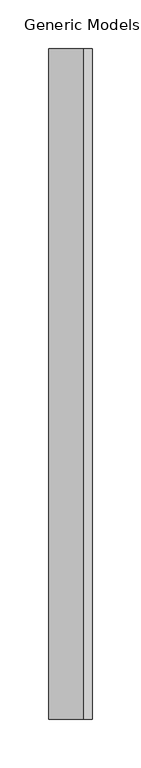
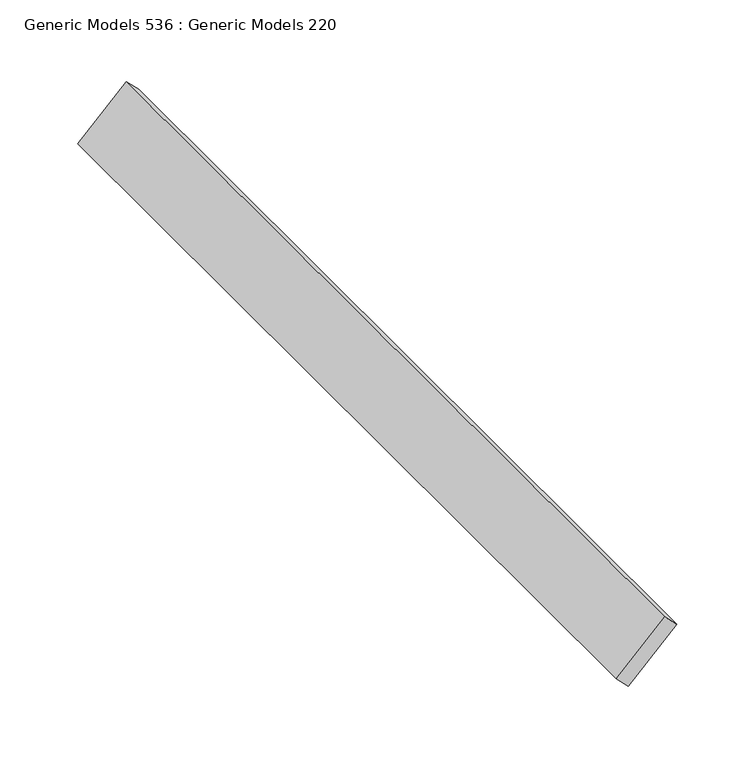
"""IFC4 building model written with IfcOpenShell, lengths in millimetres: proxy geometry, Generic Models 536 : Generic Models 220."""

from ifc_helpers import new_model, si_unit, frame, origin, place, context, project, spatial, polyline, outline, extrude, source, transform, mapped, element, save


def generic_models_536_generic_models_220_59347687(model_context):
    return source(origin(), model_context, "Body", "SweptSolid", [
        extrude(outline(polyline([(0.0, -12.7000001), (0.0, 0.0), (690.8142348, 0.0), (690.8142348, -12.7000001), (0.0, -12.7000001)])), frame((7841.3059863, 4539.4872686, 125128.6399101), z_axis=(0.7071067811868034, 0.0, 0.7071067811862918), x_axis=(0.0, -1.0, 0.0)), (0.0, 0.0, 1.0), 50.8),
    ])


if __name__ == "__main__":
    model = new_model("IFC4")
    model_context = context("Model", 3, world=origin())
    ifc_project = project(units=[si_unit("LENGTHUNIT", "METRE", prefix="MILLI")], contexts=[model_context])
    site = spatial("IfcSite", under=ifc_project)
    building = spatial("IfcBuilding", under=site)
    placement = place(None, origin())
    generic_models_536_generic_models_220_shape = generic_models_536_generic_models_220_59347687(model_context)
    element("IfcBuildingElementProxy", 1, Name="Generic Models 536 : Generic Models 220", ObjectType="Generic Models 536 : Generic Models 220", at=placement, inside=building, context=model_context, shape_type="MappedRepresentation", body=[
        mapped(generic_models_536_generic_models_220_shape, transform((0.0, 0.0, 0.0), x_axis=(1.0, 0.0, 0.0), y_axis=(0.0, 1.0, 0.0), z_axis=(0.0, 0.0, 1.0))),
    ])
    save(model, "model.ifc")

# Revit data of these elements
# Element 1 (IfcBuildingElementProxy, "Generic Models 536 : Generic Models 220")
#   Materials on its faces: "_WOOD TONE ALUMINUM EXTRUSION SLAT BY KNOTWOOD"
# Materials
#   "_WOOD TONE ALUMINUM EXTRUSION SLAT BY KNOTWOOD": class "Generic", colour RGB 177 130 114, transparency 0, Cost = 0
